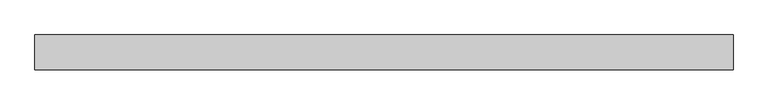
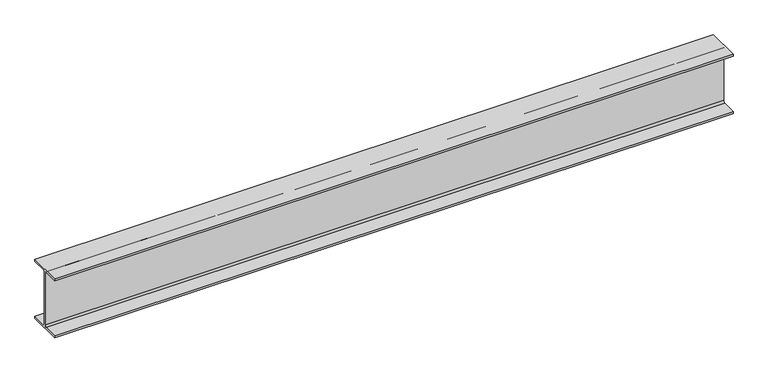
"""IFC4 building model written with IfcOpenShell, lengths in millimetres: beam geometry, Old_Steel Beam_H-KSD3502 : H_SB_ASB_H-200×200x8x12."""

from ifc_helpers import new_model, si_unit, point, frame, frame_2d, origin, place, context, project, spatial, polyline, circle_curve, trimmed, segment, composite_curve, outline, extrude, source, transform, mapped, element, save


def beam_5c7118cc(model_context):
    return source(origin(), model_context, "Body", "SweptSolid", [
        extrude(outline(composite_curve([segment(polyline([(82.5, -141.5), (82.5, -151.7), (-82.5, -151.7), (-82.5, -141.5), (-11.9, -141.5)]), True, "CONTINUOUS"), segment(trimmed(circle_curve(frame_2d((-11.9, -132.6)), 8.9), [point((-11.9, -141.5))], [point((-3.0, -132.6))], True, "CARTESIAN"), True, "CONTINUOUS"), segment(polyline([(-3.0, -132.6), (-3.0, 132.6)]), True, "CONTINUOUS"), segment(trimmed(circle_curve(frame_2d((-11.9, 132.6)), 8.9), [point((-3.0, 132.6))], [point((-11.9, 141.5))], True, "CARTESIAN"), True, "CONTINUOUS"), segment(polyline([(-11.9, 141.5), (-82.5, 141.5), (-82.5, 151.7), (82.5, 151.7), (82.5, 141.5), (11.9, 141.5)]), True, "CONTINUOUS"), segment(trimmed(circle_curve(frame_2d((11.9, 132.6)), 8.9), [point((11.9, 141.5))], [point((3.0, 132.6))], True, "CARTESIAN"), True, "CONTINUOUS"), segment(polyline([(3.0, 132.6), (3.0, -132.6)]), True, "CONTINUOUS"), segment(trimmed(circle_curve(frame_2d((11.9, -132.6)), 8.9), [point((3.0, -132.6))], [point((11.9, -141.5))], True, "CARTESIAN"), True, "CONTINUOUS"), segment(polyline([(11.9, -141.5), (82.5, -141.5)]), True, "CONTINUOUS")], self_intersect=False)), frame((-1698.1142297, 0.0, 0.0), z_axis=(1.0, 0.0, 0.0), x_axis=(0.0, 1.0, 0.0)), (0.0, 0.0, 1.0), 3290.2143671),
    ])


if __name__ == "__main__":
    model = new_model("IFC4")
    model_context = context("Model", 3, world=origin())
    ifc_project = project(units=[si_unit("LENGTHUNIT", "METRE", prefix="MILLI")], contexts=[model_context])
    site = spatial("IfcSite", under=ifc_project)
    building = spatial("IfcBuilding", under=site)
    placement = place(None, origin())
    beam_shape = beam_5c7118cc(model_context)
    element("IfcBeam", 1, ObjectType="Old_Steel Beam_H-KSD3502 : H_SB_ASB_H-200×200x8x12", at=placement, inside=building, context=model_context, shape_type="MappedRepresentation", body=[
        mapped(beam_shape, transform((0.0, 0.0, 0.0), x_axis=(1.0, 0.0, 0.0), y_axis=(0.0, 1.0, 0.0), z_axis=(0.0, 0.0, 1.0))),
    ])
    save(model, "model.ifc")

# Revit data of these elements
# Type "Old_Steel Beam_H-KSD3502 : H_SB_ASB_H-200×200x8x12"
#   Width = 20.0 cm
#   Web Thickness = 0.8 cm
#   Web Fillet = 1.3 cm
#   Warping Constant = 141376.0 cm⁶
#   Torsional Moment of Inertia = 26.2485 cm⁴
#   Torsional Modulus = 1.0 cm³
#   Section Area = 63.53 cm²
#   Plastic Modulus weak axis = 244.0 cm³
#   Plastic Modulus strong axis = 525.0 cm³
#   Perimeter = 1.16 m²/m
#   Nominal Weight = 49.90 kgf/m
#   Moment of Inertia weak axis = 1600.00 cm⁴
#   Moment of Inertia strong axis = 4720.00 cm⁴
#   Height = 20.0 cm
#   Flange Thickness = 1.2 cm
#   Elastic Modulus weak axis = 160.0 cm³
#   Elastic Modulus strong axis = 472.0 cm³
#   Centroid Vertical = 10.0 cm
#   Centroid Horizontal = 10.0 cm
#   Length [instance default] = 1.5240 m
#   Structural Material [instance default] = Steel, 45-345
#   Assembly Code = ""
# Element 1 (IfcBeam, "Old_Steel Beam_H-KSD3502 : H_SB_ASB_H-200×200x8x12")
#   Structural Material = none
# Materials
#   "Steel, 45-345": class "Metal", colour RGB 189 187 185, transparency 0, Description = "Steel 345 MPa", Cost = 0
